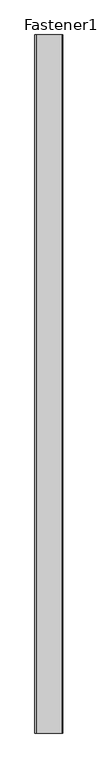
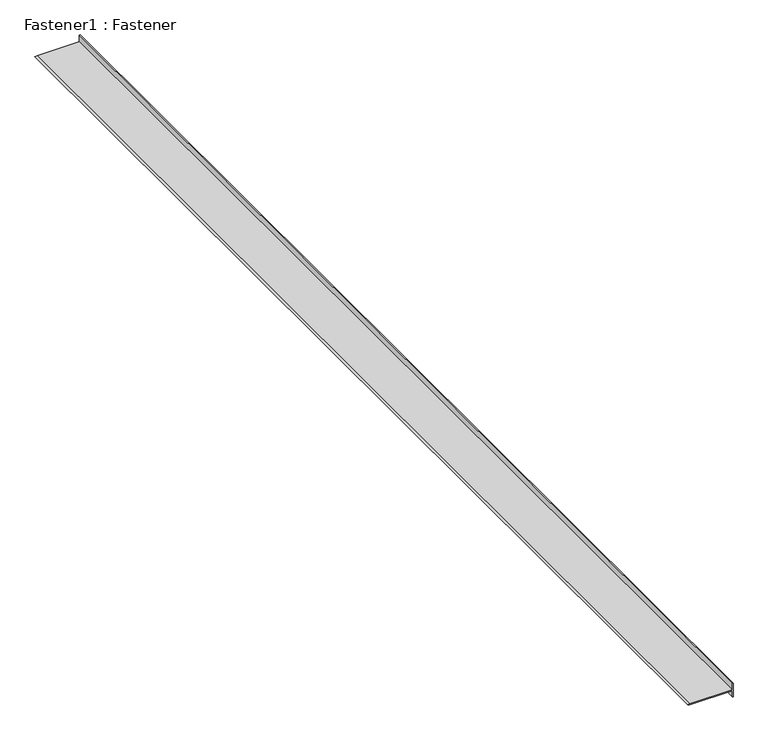
"""IFC4 building model written with IfcOpenShell, lengths in millimetres: proxy geometry, Fastener1 : Fastener."""

from ifc_helpers import new_model, si_unit, frame, origin, place, context, project, spatial, polyline, outline, extrude, source, transform, mapped, element, save


def fastener1_fastener_162db988(model_context):
    return source(origin(), model_context, "Body", "SweptSolid", [
        extrude(outline(polyline([(40087.9789725, -7085.0334918), (40113.3789725, -7085.0334918), (40113.3789725, -7086.4358356), (40101.3801444, -7086.4358356), (40101.3801444, -7161.2334918), (40100.6789725, -7165.0461872), (40099.9778006, -7161.2334918), (40099.9778006, -7086.4358356), (40087.9789725, -7086.4358356), (40087.9789725, -7085.0334918)])), frame((0.0, 7982.1531721, 0.0), z_axis=(0.0, 1.0, 0.0), x_axis=(0.0, 0.0, 1.0)), (0.0, 0.0, 1.0), 1999.85),
    ])


if __name__ == "__main__":
    model = new_model("IFC4")
    model_context = context("Model", 3, world=origin())
    ifc_project = project(units=[si_unit("LENGTHUNIT", "METRE", prefix="MILLI")], contexts=[model_context])
    site = spatial("IfcSite", under=ifc_project)
    building = spatial("IfcBuilding", under=site)
    placement = place(None, origin())
    fastener1_fastener_shape = fastener1_fastener_162db988(model_context)
    element("IfcBuildingElementProxy", 1, Name="Fastener1 : Fastener", ObjectType="Fastener1 : Fastener", at=placement, inside=building, context=model_context, shape_type="MappedRepresentation", body=[
        mapped(fastener1_fastener_shape, transform((0.0, 0.0, 0.0), x_axis=(1.0, 0.0, 0.0), y_axis=(0.0, 1.0, 0.0), z_axis=(0.0, 0.0, 1.0))),
    ])
    save(model, "model.ifc")

# Revit data of these elements
# Type "Fastener1 : Fastener"
#   NameOverride = "Fastener"
# Element 1 (IfcBuildingElementProxy, "Fastener1 : Fastener")
#   Materials on its faces: "FASTEN INTO BLOCKING"
# Materials
#   "FASTEN INTO BLOCKING": class "Unassigned", colour RGB 255 255 255, transparency 0
